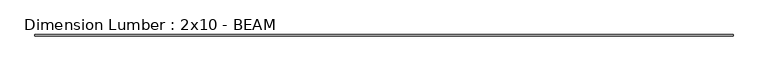
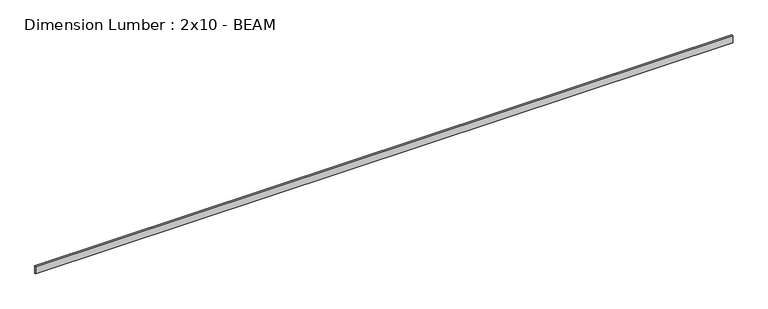
"""IFC4 building model written with IfcOpenShell, lengths in millimetres: beam geometry, Dimension Lumber : 2x10 - BEAM."""

from ifc_helpers import new_model, si_unit, frame, origin, place, context, project, spatial, polyline, outline, extrude, source, transform, mapped, element, save


def dimension_lumber_2x10_beam_42d77e94(model_context):
    return source(origin(), model_context, "Body", "SweptSolid", [
        extrude(outline(polyline([(10509.25, 19.05), (10509.25, -19.05), (-10618.7875, -19.05), (-10618.7875, 19.05), (10509.25, 19.05)])), frame((0.0, 0.0, -117.475), z_axis=(0.0, 0.0, 1.0), x_axis=(1.0, 0.0, 0.0)), (0.0, 0.0, 1.0), 234.95),
    ])


if __name__ == "__main__":
    model = new_model("IFC4")
    model_context = context("Model", 3, world=origin())
    ifc_project = project(units=[si_unit("LENGTHUNIT", "METRE", prefix="MILLI")], contexts=[model_context])
    site = spatial("IfcSite", under=ifc_project)
    building = spatial("IfcBuilding", under=site)
    placement = place(None, origin())
    dimension_lumber_2x10_beam_shape = dimension_lumber_2x10_beam_42d77e94(model_context)
    element("IfcBeam", 1, ObjectType="Dimension Lumber : 2x10 - BEAM", at=placement, inside=building, context=model_context, shape_type="MappedRepresentation", body=[
        mapped(dimension_lumber_2x10_beam_shape, transform((0.0, 0.0, 0.0), x_axis=(1.0, 0.0, 0.0), y_axis=(0.0, 1.0, 0.0), z_axis=(0.0, 0.0, 1.0))),
    ])
    save(model, "model.ifc")

# Revit data of these elements
# Type "Dimension Lumber : 2x10 - BEAM"
#   Assembly Code = "B10"
#   A = 0.0755556 SF
#   Length [instance default] = 5' - 0"
#   b = 0' - 1 1/2"
#   d = 0' - 9 1/4"
#   Structural Material = (3) SISTERED 2X10s AT BEAM
# Element 1 (IfcBeam, "Dimension Lumber : 2x10 - BEAM")
#   Materials on its faces: "(3) SISTERED 2X10s AT BEAM"
# Materials
#   "(3) SISTERED 2X10s AT BEAM": class "Wood", colour RGB 234 198 147, transparency 0, Description = "Pinus Echinata", Cost = 0
